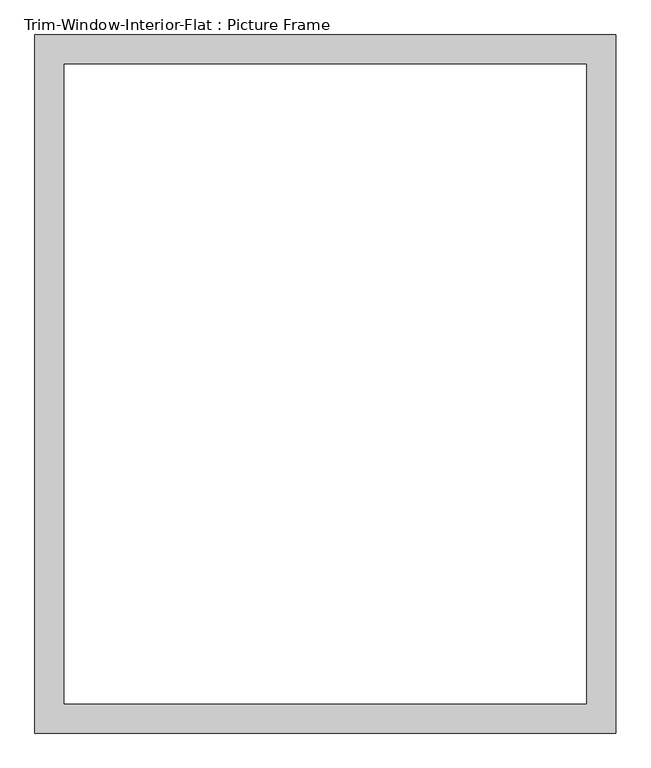
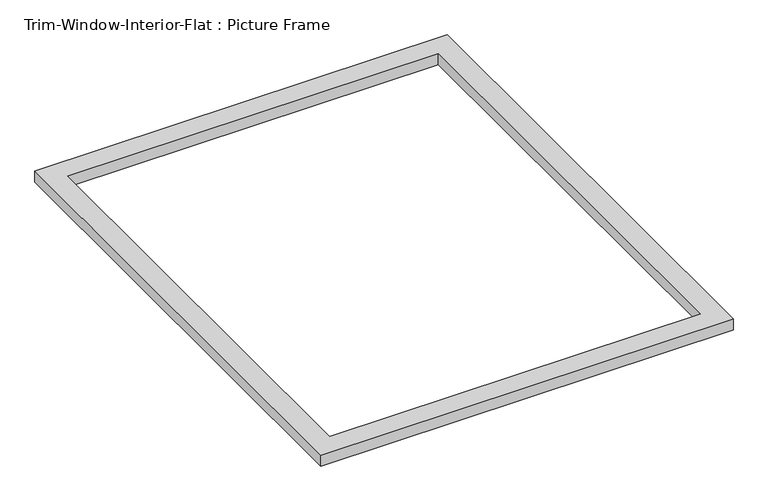
"""IFC4 building model written with IfcOpenShell, lengths in millimetres: proxy geometry, Trim-Window-Interior-Flat : Picture Frame."""

import ifcopenshell
import ifcopenshell.guid

model = None  # the IFC model being written
_history = None  # IfcOwnerHistory: only IFC2X3 demands one
_inside = {}  # id of a spatial element -> (the spatial element, [elements in it])
_under = {}  # id of a project, library or spatial element -> (it, [spatial elements below it])
_declared = {}  # id of a project -> (the project, [libraries it declares])
_typed = {}  # id of a type object -> (the type object, [elements of that type])
_made_of = {}  # id of a material, layer set ... -> (it, [elements and type objects made of it])


def new_model(schema):
    """Start an empty IFC model of exactly this schema.

    Asked for "IFC4X3", IfcOpenShell would pick the latest addendum, in which some entities
    have other attributes; the version numbers below select the first issue.
    IFC2X3 requires an IfcOwnerHistory on every rooted entity: one is made here for all.
    """
    global model, _history
    if schema == "IFC4X3":
        model = ifcopenshell.file(schema_version=(4, 3, 0, 0))
    else:
        model = ifcopenshell.file(schema=schema)
    _inside.clear()
    _under.clear()
    _declared.clear()
    _typed.clear()
    _made_of.clear()
    _history = None
    if model.schema == "IFC2X3":
        org = make("IfcOrganization", Name="unknown")
        user = make(
            "IfcPersonAndOrganization",
            ThePerson=make("IfcPerson", FamilyName="unknown"),
            TheOrganization=org,
        )
        app = make(
            "IfcApplication",
            ApplicationDeveloper=org,
            Version="unknown",
            ApplicationFullName="unknown",
            ApplicationIdentifier="unknown",
        )
        _history = make(
            "IfcOwnerHistory",
            OwningUser=user,
            OwningApplication=app,
            ChangeAction="ADDED",
            CreationDate=0,
        )
    return model


def make(cls, **values):
    """One entity of the class cls with the attributes given. An attribute that is None is left unset."""
    return model.create_entity(
        cls, **{name: value for name, value in values.items() if value is not None}
    )


def rooted(cls, **values):
    """An entity with a GlobalId (a new one), such as an element, a storey or a relation."""
    return make(cls, GlobalId=ifcopenshell.guid.new(), OwnerHistory=_history, **values)


def si_unit(unit_type, name, prefix=None):
    """IfcSIUnit, for example si_unit("LENGTHUNIT", "METRE", prefix="MILLI")."""
    return make("IfcSIUnit", UnitType=unit_type, Prefix=prefix, Name=name)


def assignment(units):
    """IfcUnitAssignment: the units of a project."""
    return None if units is None else make("IfcUnitAssignment", Units=units)


def point(xyz):
    """IfcCartesianPoint."""
    return None if xyz is None else make("IfcCartesianPoint", Coordinates=xyz)


def direction(xyz):
    """IfcDirection."""
    return None if xyz is None else make("IfcDirection", DirectionRatios=xyz)


def frame(location, z_axis=None, x_axis=None):
    """IfcAxis2Placement3D, a coordinate frame: its origin and axes. An axis left out is left unset."""
    return make(
        "IfcAxis2Placement3D",
        Location=point(location),
        Axis=direction(z_axis),
        RefDirection=direction(x_axis),
    )


def origin():
    """The frame at (0, 0, 0) with its axes left unset."""
    return frame((0.0, 0.0, 0.0))


def origin_with_axes():
    """The frame at (0, 0, 0) with the z axis (0, 0, 1) and the x axis (1, 0, 0) written out."""
    return frame((0.0, 0.0, 0.0), z_axis=(0.0, 0.0, 1.0), x_axis=(1.0, 0.0, 0.0))


def place(relative_to, where):
    """IfcLocalPlacement: puts the frame where relative to a parent placement (None: the world)."""
    return make(
        "IfcLocalPlacement", PlacementRelTo=relative_to, RelativePlacement=where
    )


def context(
    kind, dimensions, precision=None, world=None, true_north=None, identifier=None
):
    """IfcGeometricRepresentationContext, for example the 3D "Model" context."""
    return make(
        "IfcGeometricRepresentationContext",
        ContextIdentifier=identifier,
        ContextType=kind,
        CoordinateSpaceDimension=dimensions,
        Precision=precision,
        WorldCoordinateSystem=world,
        TrueNorth=true_north,
    )


def project(units=None, contexts=None):
    """IfcProject with its units and contexts."""
    return rooted(
        "IfcProject",
        Name="project",
        RepresentationContexts=contexts,
        UnitsInContext=assignment(units),
    )


def spatial(cls, under=None, at=None, **own):
    """A site, building, storey or space (cls), placed at a placement, below another one or the project."""
    s = rooted(cls, ObjectPlacement=at, **own)
    if under is not None:
        _under.setdefault(under.id(), (under, []))[1].append(s)
    return s


def polyline(points):
    """IfcPolyline through the points."""
    return make("IfcPolyline", Points=[point(p) for p in points])


def outline(outer, holes=None, kind="AREA"):
    """IfcArbitraryClosedProfileDef: a profile drawn as a closed curve; with holes, ...WithVoids."""
    if holes is None:
        return make("IfcArbitraryClosedProfileDef", ProfileType=kind, OuterCurve=outer)
    return make(
        "IfcArbitraryProfileDefWithVoids",
        ProfileType=kind,
        OuterCurve=outer,
        InnerCurves=holes,
    )


def extrude(swept, where, along, depth):
    """IfcExtrudedAreaSolid: the profile swept, set in the frame where, extruded along a direction by depth."""
    return make(
        "IfcExtrudedAreaSolid",
        SweptArea=swept,
        Position=where,
        ExtrudedDirection=direction(along),
        Depth=depth,
    )


def shape(context_of_items, identifier, shape_type, items):
    """IfcShapeRepresentation: the items that make up one representation, for example the "Body"."""
    return make(
        "IfcShapeRepresentation",
        ContextOfItems=context_of_items,
        RepresentationIdentifier=identifier,
        RepresentationType=shape_type,
        Items=items,
    )


def source(mapping_origin, context_of_items, identifier, shape_type, items):
    """IfcRepresentationMap: a shape defined once, which mapped items show again and again."""
    return make(
        "IfcRepresentationMap",
        MappingOrigin=mapping_origin,
        MappedRepresentation=shape(context_of_items, identifier, shape_type, items),
    )


def transform(
    local_origin,
    x_axis=None,
    y_axis=None,
    z_axis=None,
    scale=None,
    scale2=None,
    scale3=None,
    uniform=True,
):
    """IfcCartesianTransformationOperator3D, or its non-uniform kind. x_axis, y_axis, z_axis: its Axis1, 2, 3."""
    if uniform:
        return make(
            "IfcCartesianTransformationOperator3D",
            Axis1=direction(x_axis),
            Axis2=direction(y_axis),
            LocalOrigin=point(local_origin),
            Scale=scale,
            Axis3=direction(z_axis),
        )
    return make(
        "IfcCartesianTransformationOperator3DnonUniform",
        Axis1=direction(x_axis),
        Axis2=direction(y_axis),
        LocalOrigin=point(local_origin),
        Scale=scale,
        Axis3=direction(z_axis),
        Scale2=scale2,
        Scale3=scale3,
    )


def mapped(mapping_source, mapping_target):
    """IfcMappedItem: shows the shape of a source again, moved by a transform."""
    return make(
        "IfcMappedItem", MappingSource=mapping_source, MappingTarget=mapping_target
    )


def made_of(thing, what):
    """Note that an element or type object is made of a material, layer set ...; save() writes the relation."""
    if what is not None:
        _made_of.setdefault(what.id(), (what, []))[1].append(thing)
    return thing


def element(
    cls,
    number,
    at=None,
    inside=None,
    cuts=None,
    type_object=None,
    material=None,
    context=None,
    identifier="Body",
    shape_type=None,
    held_by="IfcProductDefinitionShape",
    body=None,
    shapes=None,
    **own,
):
    """One element of the class cls, such as IfcWall. Its Tag is "e" and its number.

    at: its placement. inside: the storey or other place that contains it. cuts: it is an
    opening in that element (IfcRelVoidsElement). A single representation is given by context,
    identifier, shape_type and body (its items); several are given by shapes. held_by: the class
    of the entity that holds the representations. save() writes the other relations.
    """
    e = rooted(cls, Tag="e%d" % number, ObjectPlacement=at, **own)
    if body is not None:
        shapes = [shape(context, identifier, shape_type, body)]
    if shapes is not None:
        e.Representation = make(held_by, Representations=shapes)
    if inside is not None:
        _inside.setdefault(inside.id(), (inside, []))[1].append(e)
    if cuts is not None:
        rooted(
            "IfcRelVoidsElement", RelatingBuildingElement=cuts, RelatedOpeningElement=e
        )
    if type_object is not None:
        _typed.setdefault(type_object.id(), (type_object, []))[1].append(e)
    return made_of(e, material)


def aggregate(whole, parts):
    """IfcRelAggregates: a whole, such as a stair, and the parts it consists of."""
    return rooted("IfcRelAggregates", RelatingObject=whole, RelatedObjects=parts)


def save(model, path):
    """Write the relations noted so far, then the file.

    IfcRelAggregates (storeys below a building ...), IfcRelContainedInSpatialStructure (elements
    in a storey), IfcRelDefinesByType, IfcRelAssociatesMaterial and IfcRelDeclares: one each for
    every whole, place, type object, material and project.
    """
    for whole, parts in _under.values():
        aggregate(whole, parts)
    for where, things in _inside.values():
        rooted(
            "IfcRelContainedInSpatialStructure",
            RelatedElements=things,
            RelatingStructure=where,
        )
    for kind, things in _typed.values():
        rooted("IfcRelDefinesByType", RelatedObjects=things, RelatingType=kind)
    for what, things in _made_of.values():
        rooted("IfcRelAssociatesMaterial", RelatedObjects=things, RelatingMaterial=what)
    for by, libraries in _declared.values():
        rooted("IfcRelDeclares", RelatingContext=by, RelatedDefinitions=libraries)
    model.write(path)


def trim_window_interior_flat_picture_frame_75e883e6(model_context):
    return source(origin(), model_context, "Body", "SweptSolid", [
        extrude(outline(polyline([(565.15, -44.45), (-565.15, -44.45), (-565.15, 1314.45), (565.15, 1314.45), (565.15, -44.45)]), holes=[polyline([(508.0, 12.7), (508.0, 1257.3), (-508.0, 1257.3), (-508.0, 12.7), (508.0, 12.7)])]), origin_with_axes(), (0.0, 0.0, 1.0), 31.75),
    ])


if __name__ == "__main__":
    model = new_model("IFC4")
    model_context = context("Model", 3, world=origin())
    ifc_project = project(units=[si_unit("LENGTHUNIT", "METRE", prefix="MILLI")], contexts=[model_context])
    site = spatial("IfcSite", under=ifc_project)
    building = spatial("IfcBuilding", under=site)
    placement = place(None, origin())
    trim_window_interior_flat_picture_frame_shape = trim_window_interior_flat_picture_frame_75e883e6(model_context)
    element("IfcBuildingElementProxy", 1, Name="Trim-Window-Interior-Flat : Picture Frame", ObjectType="Trim-Window-Interior-Flat : Picture Frame", at=placement, inside=building, context=model_context, shape_type="MappedRepresentation", body=[
        mapped(trim_window_interior_flat_picture_frame_shape, transform((0.0, 0.0, 0.0), x_axis=(1.0, 0.0, 0.0), y_axis=(0.0, 1.0, 0.0), z_axis=(0.0, 0.0, 1.0))),
    ])
    save(model, "model.ifc")

# Revit data of these elements
# Type "Trim-Window-Interior-Flat : Picture Frame"
#   Trim Thickness_Picture Frame = 0' - 1 1/4"
#   Trim Width = 0' - 2 1/4"
#   Trim Thickness_with Sill = 0' - 0 3/4"
#   Sill Thickness = 0' - 1 1/4"
#   Opening Width [instance default] = 2' - 0"
#   Opening Height [instance default] = 3' - 0"
#   Default Elevation = 4' - 0"
#   Sill = no
#   Picture Frame = yes
#   Trim Material [instance default] = none
# Element 1 (IfcBuildingElementProxy, "Trim-Window-Interior-Flat : Picture Frame")
#   Opening Width = 3' - 5"
#   Opening Height = 4' - 2"
#   Trim Material = Wood - Stained
#   Materials on its faces: "Wood - Stained"
# Materials
#   "Wood - Stained": class "Wood", colour RGB 224 178 126, transparency 0, Cost = 0
